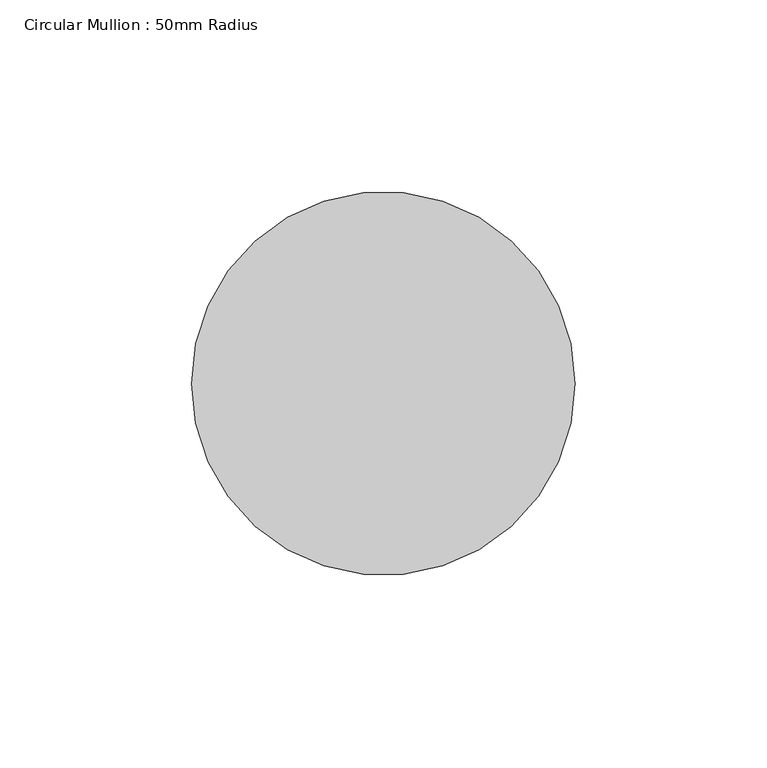
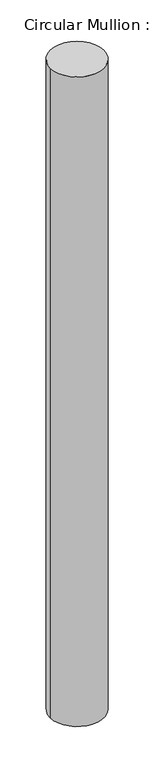
"""IFC4 building model written with IfcOpenShell, lengths in millimetres: member geometry, Circular Mullion : 50mm Radius."""

from ifc_helpers import new_model, si_unit, point, frame, origin, origin_2d, place, context, project, spatial, circle_curve, trimmed, segment, composite_curve, outline, extrude, source, transform, mapped, element, save


def circular_mullion_50mm_radius_a78e111e(model_context):
    return source(origin(), model_context, "Body", "SweptSolid", [
        extrude(outline(composite_curve([segment(trimmed(circle_curve(origin_2d(), 50.0), [point((50.0, 0.0))], [point((-50.0, 0.0))], False, "CARTESIAN"), True, "CONTINUOUS"), segment(trimmed(circle_curve(origin_2d(), 50.0), [point((-50.0, 0.0))], [point((50.0, 0.0))], False, "CARTESIAN"), True, "CONTINUOUS")], self_intersect=False)), frame((0.0, 0.0, -1279.3133782), z_axis=(0.0, 0.0, 1.0), x_axis=(1.0, 0.0, 0.0)), (0.0, 0.0, 1.0), 1279.3133782),
    ])


if __name__ == "__main__":
    model = new_model("IFC4")
    model_context = context("Model", 3, world=origin())
    ifc_project = project(units=[si_unit("LENGTHUNIT", "METRE", prefix="MILLI")], contexts=[model_context])
    site = spatial("IfcSite", under=ifc_project)
    building = spatial("IfcBuilding", under=site)
    placement = place(None, origin())
    circular_mullion_50mm_radius_shape = circular_mullion_50mm_radius_a78e111e(model_context)
    element("IfcMember", 1, ObjectType="Circular Mullion : 50mm Radius", at=placement, inside=building, context=model_context, shape_type="MappedRepresentation", body=[
        mapped(circular_mullion_50mm_radius_shape, transform((0.0, 0.0, 0.0), x_axis=(1.0, 0.0, 0.0), y_axis=(0.0, 1.0, 0.0), z_axis=(0.0, 0.0, 1.0))),
    ])
    save(model, "model.ifc")

# Revit data of these elements
# Type "Circular Mullion : 50mm Radius"
#   built-in parameter 1007350 = 0.164042 (stored number, unit not read)
# Element 1 (IfcMember, "Circular Mullion : 50mm Radius")
#   Materials on its faces: "Aluminium"
# Materials
#   "Aluminium": class "Metal", colour RGB 247 247 247, transparency 0, Description = "Aluminium 6061", Cost = 0
